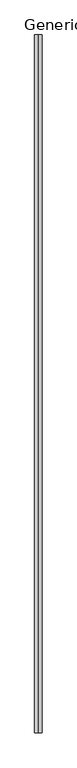
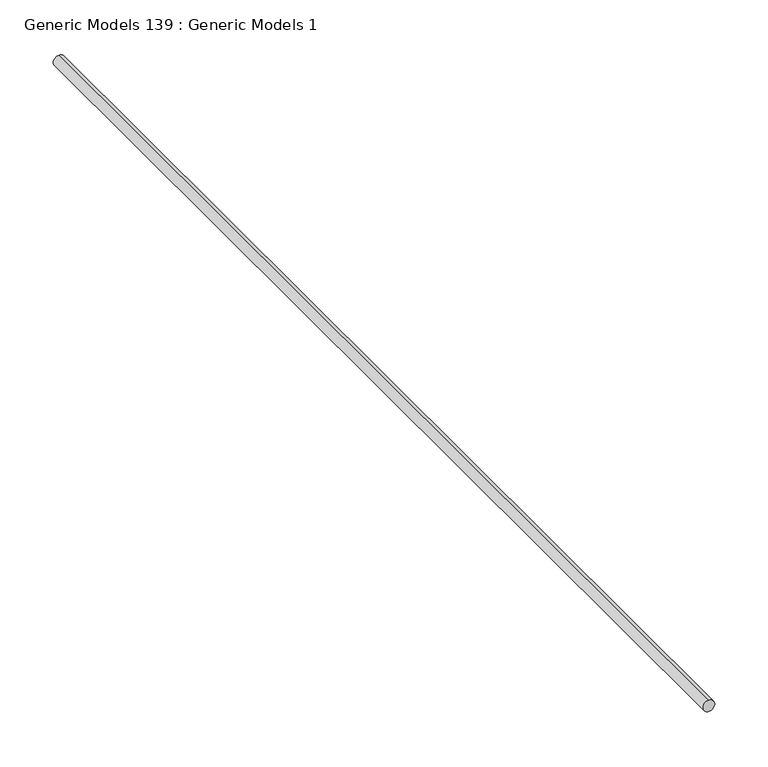
"""IFC4 building model written with IfcOpenShell, lengths in millimetres: proxy geometry, Generic Models 139 : Generic Models 1."""

from ifc_helpers import new_model, si_unit, point, frame, frame_2d, origin, place, context, project, spatial, circle_curve, trimmed, segment, composite_curve, outline, extrude, source, transform, mapped, element, save


def generic_models_139_generic_models_1_e596f594(model_context):
    return source(origin(), model_context, "Body", "SweptSolid", [
        extrude(outline(composite_curve([segment(trimmed(circle_curve(frame_2d((97.5288266, 52112.9548165)), 6.35), [point((91.1788266, 52112.9548165))], [point((103.8788266, 52112.9548165))], False, "CARTESIAN"), True, "CONTINUOUS"), segment(trimmed(circle_curve(frame_2d((97.5288266, 52112.9548165)), 6.35), [point((103.8788266, 52112.9548165))], [point((91.1788266, 52112.9548165))], False, "CARTESIAN"), True, "CONTINUOUS")], self_intersect=False)), frame((0.0, 0.0, 0.0), z_axis=(0.0, 1.0, 0.0), x_axis=(0.0, 0.0, 1.0)), (0.0, 0.0, 1.0), 1219.2),
    ])


if __name__ == "__main__":
    model = new_model("IFC4")
    model_context = context("Model", 3, world=origin())
    ifc_project = project(units=[si_unit("LENGTHUNIT", "METRE", prefix="MILLI")], contexts=[model_context])
    site = spatial("IfcSite", under=ifc_project)
    building = spatial("IfcBuilding", under=site)
    placement = place(None, origin())
    generic_models_139_generic_models_1_shape = generic_models_139_generic_models_1_e596f594(model_context)
    element("IfcBuildingElementProxy", 1, Name="Generic Models 139 : Generic Models 1", ObjectType="Generic Models 139 : Generic Models 1", at=placement, inside=building, context=model_context, shape_type="MappedRepresentation", body=[
        mapped(generic_models_139_generic_models_1_shape, transform((0.0, 0.0, 0.0), x_axis=(1.0, 0.0, 0.0), y_axis=(0.0, 1.0, 0.0), z_axis=(0.0, 0.0, 1.0))),
    ])
    save(model, "model.ifc")

# Revit data of these elements
# Element 1 (IfcBuildingElementProxy, "Generic Models 139 : Generic Models 1")
#   Materials on its faces: "#4 CONT. STEEL REBAR"
# Materials
#   "#4 CONT. STEEL REBAR": class "Metal", colour RGB 189 187 185, transparency 0, Description = "Structural steel 50ksi", Cost = 0
